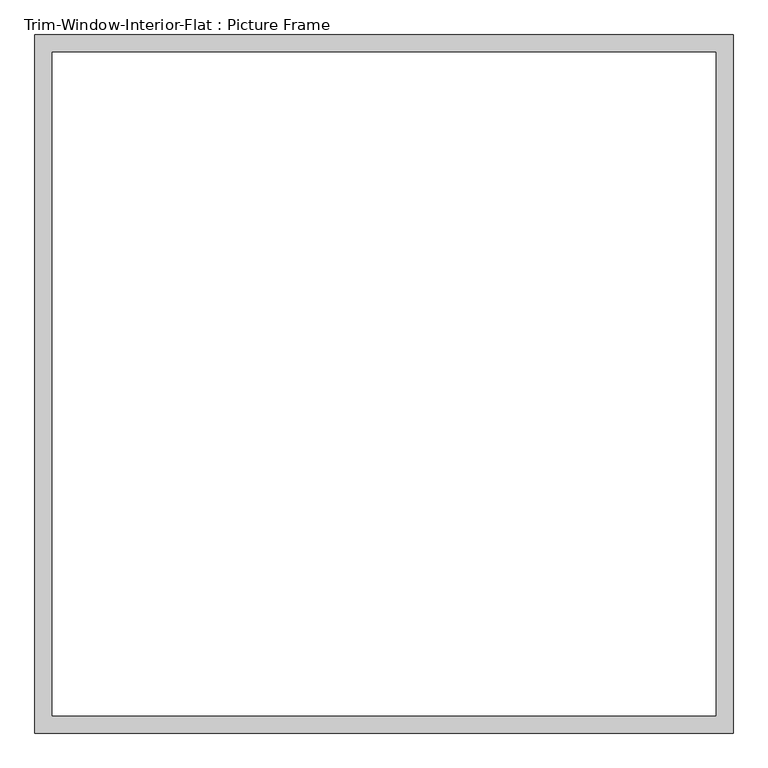
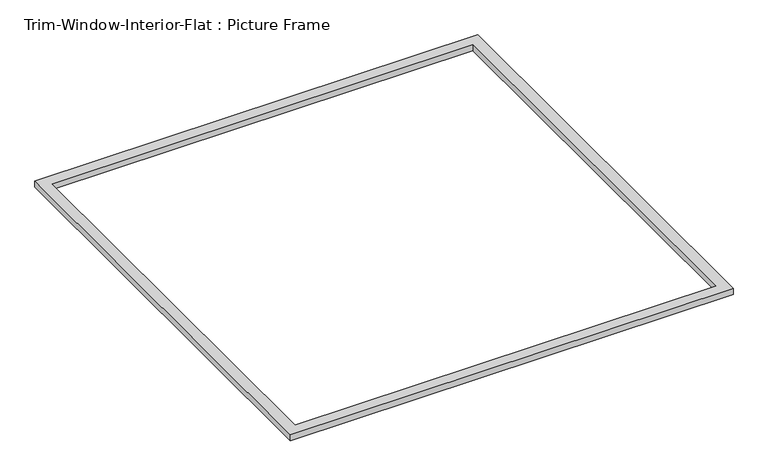
"""IFC4 building model written with IfcOpenShell, lengths in millimetres: proxy geometry, Trim-Window-Interior-Flat : Picture Frame."""

import ifcopenshell
import ifcopenshell.guid

model = None  # the IFC model being written
_history = None  # IfcOwnerHistory: only IFC2X3 demands one
_inside = {}  # id of a spatial element -> (the spatial element, [elements in it])
_under = {}  # id of a project, library or spatial element -> (it, [spatial elements below it])
_declared = {}  # id of a project -> (the project, [libraries it declares])
_typed = {}  # id of a type object -> (the type object, [elements of that type])
_made_of = {}  # id of a material, layer set ... -> (it, [elements and type objects made of it])


def new_model(schema):
    """Start an empty IFC model of exactly this schema.

    Asked for "IFC4X3", IfcOpenShell would pick the latest addendum, in which some entities
    have other attributes; the version numbers below select the first issue.
    IFC2X3 requires an IfcOwnerHistory on every rooted entity: one is made here for all.
    """
    global model, _history
    if schema == "IFC4X3":
        model = ifcopenshell.file(schema_version=(4, 3, 0, 0))
    else:
        model = ifcopenshell.file(schema=schema)
    _inside.clear()
    _under.clear()
    _declared.clear()
    _typed.clear()
    _made_of.clear()
    _history = None
    if model.schema == "IFC2X3":
        org = make("IfcOrganization", Name="unknown")
        user = make(
            "IfcPersonAndOrganization",
            ThePerson=make("IfcPerson", FamilyName="unknown"),
            TheOrganization=org,
        )
        app = make(
            "IfcApplication",
            ApplicationDeveloper=org,
            Version="unknown",
            ApplicationFullName="unknown",
            ApplicationIdentifier="unknown",
        )
        _history = make(
            "IfcOwnerHistory",
            OwningUser=user,
            OwningApplication=app,
            ChangeAction="ADDED",
            CreationDate=0,
        )
    return model


def make(cls, **values):
    """One entity of the class cls with the attributes given. An attribute that is None is left unset."""
    return model.create_entity(
        cls, **{name: value for name, value in values.items() if value is not None}
    )


def rooted(cls, **values):
    """An entity with a GlobalId (a new one), such as an element, a storey or a relation."""
    return make(cls, GlobalId=ifcopenshell.guid.new(), OwnerHistory=_history, **values)


def si_unit(unit_type, name, prefix=None):
    """IfcSIUnit, for example si_unit("LENGTHUNIT", "METRE", prefix="MILLI")."""
    return make("IfcSIUnit", UnitType=unit_type, Prefix=prefix, Name=name)


def assignment(units):
    """IfcUnitAssignment: the units of a project."""
    return None if units is None else make("IfcUnitAssignment", Units=units)


def point(xyz):
    """IfcCartesianPoint."""
    return None if xyz is None else make("IfcCartesianPoint", Coordinates=xyz)


def direction(xyz):
    """IfcDirection."""
    return None if xyz is None else make("IfcDirection", DirectionRatios=xyz)


def frame(location, z_axis=None, x_axis=None):
    """IfcAxis2Placement3D, a coordinate frame: its origin and axes. An axis left out is left unset."""
    return make(
        "IfcAxis2Placement3D",
        Location=point(location),
        Axis=direction(z_axis),
        RefDirection=direction(x_axis),
    )


def origin():
    """The frame at (0, 0, 0) with its axes left unset."""
    return frame((0.0, 0.0, 0.0))


def origin_with_axes():
    """The frame at (0, 0, 0) with the z axis (0, 0, 1) and the x axis (1, 0, 0) written out."""
    return frame((0.0, 0.0, 0.0), z_axis=(0.0, 0.0, 1.0), x_axis=(1.0, 0.0, 0.0))


def place(relative_to, where):
    """IfcLocalPlacement: puts the frame where relative to a parent placement (None: the world)."""
    return make(
        "IfcLocalPlacement", PlacementRelTo=relative_to, RelativePlacement=where
    )


def context(
    kind, dimensions, precision=None, world=None, true_north=None, identifier=None
):
    """IfcGeometricRepresentationContext, for example the 3D "Model" context."""
    return make(
        "IfcGeometricRepresentationContext",
        ContextIdentifier=identifier,
        ContextType=kind,
        CoordinateSpaceDimension=dimensions,
        Precision=precision,
        WorldCoordinateSystem=world,
        TrueNorth=true_north,
    )


def project(units=None, contexts=None):
    """IfcProject with its units and contexts."""
    return rooted(
        "IfcProject",
        Name="project",
        RepresentationContexts=contexts,
        UnitsInContext=assignment(units),
    )


def spatial(cls, under=None, at=None, **own):
    """A site, building, storey or space (cls), placed at a placement, below another one or the project."""
    s = rooted(cls, ObjectPlacement=at, **own)
    if under is not None:
        _under.setdefault(under.id(), (under, []))[1].append(s)
    return s


def polyline(points):
    """IfcPolyline through the points."""
    return make("IfcPolyline", Points=[point(p) for p in points])


def outline(outer, holes=None, kind="AREA"):
    """IfcArbitraryClosedProfileDef: a profile drawn as a closed curve; with holes, ...WithVoids."""
    if holes is None:
        return make("IfcArbitraryClosedProfileDef", ProfileType=kind, OuterCurve=outer)
    return make(
        "IfcArbitraryProfileDefWithVoids",
        ProfileType=kind,
        OuterCurve=outer,
        InnerCurves=holes,
    )


def extrude(swept, where, along, depth):
    """IfcExtrudedAreaSolid: the profile swept, set in the frame where, extruded along a direction by depth."""
    return make(
        "IfcExtrudedAreaSolid",
        SweptArea=swept,
        Position=where,
        ExtrudedDirection=direction(along),
        Depth=depth,
    )


def shape(context_of_items, identifier, shape_type, items):
    """IfcShapeRepresentation: the items that make up one representation, for example the "Body"."""
    return make(
        "IfcShapeRepresentation",
        ContextOfItems=context_of_items,
        RepresentationIdentifier=identifier,
        RepresentationType=shape_type,
        Items=items,
    )


def source(mapping_origin, context_of_items, identifier, shape_type, items):
    """IfcRepresentationMap: a shape defined once, which mapped items show again and again."""
    return make(
        "IfcRepresentationMap",
        MappingOrigin=mapping_origin,
        MappedRepresentation=shape(context_of_items, identifier, shape_type, items),
    )


def transform(
    local_origin,
    x_axis=None,
    y_axis=None,
    z_axis=None,
    scale=None,
    scale2=None,
    scale3=None,
    uniform=True,
):
    """IfcCartesianTransformationOperator3D, or its non-uniform kind. x_axis, y_axis, z_axis: its Axis1, 2, 3."""
    if uniform:
        return make(
            "IfcCartesianTransformationOperator3D",
            Axis1=direction(x_axis),
            Axis2=direction(y_axis),
            LocalOrigin=point(local_origin),
            Scale=scale,
            Axis3=direction(z_axis),
        )
    return make(
        "IfcCartesianTransformationOperator3DnonUniform",
        Axis1=direction(x_axis),
        Axis2=direction(y_axis),
        LocalOrigin=point(local_origin),
        Scale=scale,
        Axis3=direction(z_axis),
        Scale2=scale2,
        Scale3=scale3,
    )


def mapped(mapping_source, mapping_target):
    """IfcMappedItem: shows the shape of a source again, moved by a transform."""
    return make(
        "IfcMappedItem", MappingSource=mapping_source, MappingTarget=mapping_target
    )


def made_of(thing, what):
    """Note that an element or type object is made of a material, layer set ...; save() writes the relation."""
    if what is not None:
        _made_of.setdefault(what.id(), (what, []))[1].append(thing)
    return thing


def element(
    cls,
    number,
    at=None,
    inside=None,
    cuts=None,
    type_object=None,
    material=None,
    context=None,
    identifier="Body",
    shape_type=None,
    held_by="IfcProductDefinitionShape",
    body=None,
    shapes=None,
    **own,
):
    """One element of the class cls, such as IfcWall. Its Tag is "e" and its number.

    at: its placement. inside: the storey or other place that contains it. cuts: it is an
    opening in that element (IfcRelVoidsElement). A single representation is given by context,
    identifier, shape_type and body (its items); several are given by shapes. held_by: the class
    of the entity that holds the representations. save() writes the other relations.
    """
    e = rooted(cls, Tag="e%d" % number, ObjectPlacement=at, **own)
    if body is not None:
        shapes = [shape(context, identifier, shape_type, body)]
    if shapes is not None:
        e.Representation = make(held_by, Representations=shapes)
    if inside is not None:
        _inside.setdefault(inside.id(), (inside, []))[1].append(e)
    if cuts is not None:
        rooted(
            "IfcRelVoidsElement", RelatingBuildingElement=cuts, RelatedOpeningElement=e
        )
    if type_object is not None:
        _typed.setdefault(type_object.id(), (type_object, []))[1].append(e)
    return made_of(e, material)


def aggregate(whole, parts):
    """IfcRelAggregates: a whole, such as a stair, and the parts it consists of."""
    return rooted("IfcRelAggregates", RelatingObject=whole, RelatedObjects=parts)


def save(model, path):
    """Write the relations noted so far, then the file.

    IfcRelAggregates (storeys below a building ...), IfcRelContainedInSpatialStructure (elements
    in a storey), IfcRelDefinesByType, IfcRelAssociatesMaterial and IfcRelDeclares: one each for
    every whole, place, type object, material and project.
    """
    for whole, parts in _under.values():
        aggregate(whole, parts)
    for where, things in _inside.values():
        rooted(
            "IfcRelContainedInSpatialStructure",
            RelatedElements=things,
            RelatingStructure=where,
        )
    for kind, things in _typed.values():
        rooted("IfcRelDefinesByType", RelatedObjects=things, RelatingType=kind)
    for what, things in _made_of.values():
        rooted("IfcRelAssociatesMaterial", RelatedObjects=things, RelatingMaterial=what)
    for by, libraries in _declared.values():
        rooted("IfcRelDeclares", RelatingContext=by, RelatedDefinitions=libraries)
    model.write(path)


def trim_window_interior_flat_picture_frame_c49be291(model_context):
    return source(origin(), model_context, "Body", "SweptSolid", [
        extrude(outline(polyline([(1144.45, 44.45), (1144.45, -2244.45), (-1144.45, -2244.45), (-1144.45, 44.45), (1144.45, 44.45)]), holes=[polyline([(1087.3, -12.7), (-1087.3, -12.7), (-1087.3, -2187.3), (1087.3, -2187.3), (1087.3, -12.7)])]), origin_with_axes(), (0.0, 0.0, 1.0), 31.75),
    ])


if __name__ == "__main__":
    model = new_model("IFC4")
    model_context = context("Model", 3, world=origin())
    ifc_project = project(units=[si_unit("LENGTHUNIT", "METRE", prefix="MILLI")], contexts=[model_context])
    site = spatial("IfcSite", under=ifc_project)
    building = spatial("IfcBuilding", under=site)
    placement = place(None, origin())
    trim_window_interior_flat_picture_frame_shape = trim_window_interior_flat_picture_frame_c49be291(model_context)
    element("IfcBuildingElementProxy", 1, Name="Trim-Window-Interior-Flat : Picture Frame", ObjectType="Trim-Window-Interior-Flat : Picture Frame", at=placement, inside=building, context=model_context, shape_type="MappedRepresentation", body=[
        mapped(trim_window_interior_flat_picture_frame_shape, transform((0.0, 0.0, 0.0), x_axis=(1.0, 0.0, 0.0), y_axis=(0.0, 1.0, 0.0), z_axis=(0.0, 0.0, 1.0))),
    ])
    save(model, "model.ifc")

# Revit data of these elements
# Type "Trim-Window-Interior-Flat : Picture Frame"
#   Trim Thickness_Picture Frame = 0.03175 m
#   Trim Width = 0.05715 m
#   Trim Thickness_with Sill = 0.01905 m
#   Sill Thickness = 0.03175 m
#   Opening Width [instance default] = 0.6096 m
#   Opening Height [instance default] = 0.9144 m
#   Default Elevation = 1.2192 m
#   Sill = no
#   Picture Frame = yes
#   Trim Material [instance default] = none
# Element 1 (IfcBuildingElementProxy, "Trim-Window-Interior-Flat : Picture Frame")
#   Opening Width = 2.2 m
#   Opening Height = 2.2 m
#   Trim Material = Wood - Stained
#   Materials on its faces: "Wood - Stained"
# Materials
#   "Wood - Stained": class "Wood", colour RGB 227 170 128, transparency 0, Cost = 0
